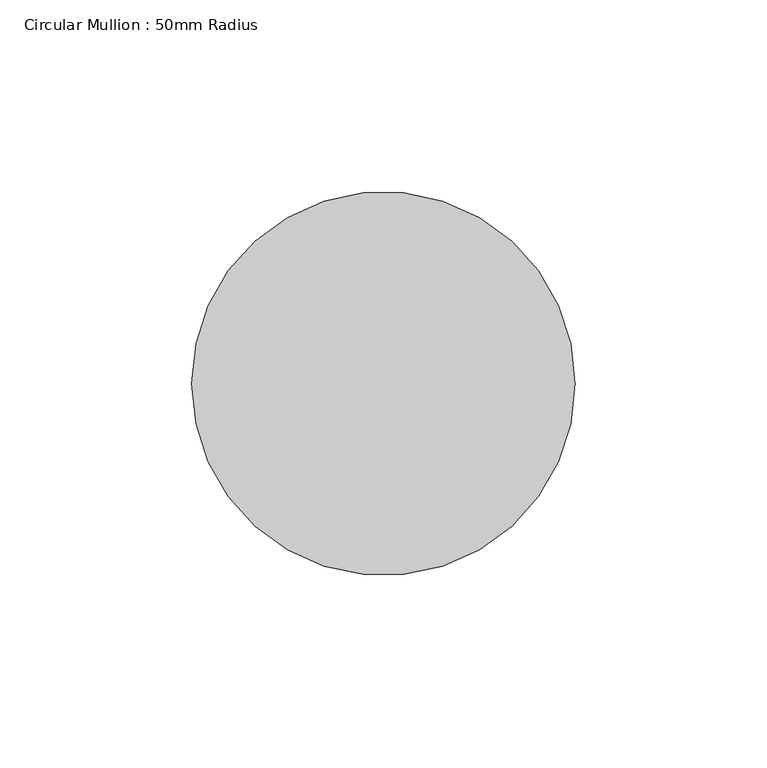
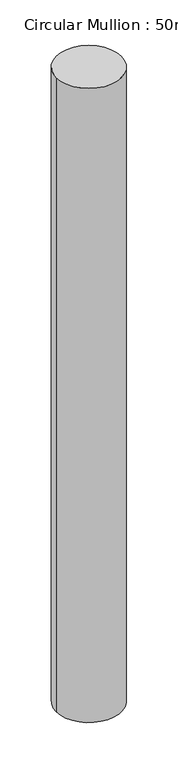
"""IFC4 building model written with IfcOpenShell, lengths in millimetres: member geometry, Circular Mullion : 50mm Radius."""

from ifc_helpers import new_model, si_unit, point, frame, origin, origin_2d, place, context, project, spatial, circle_curve, trimmed, segment, composite_curve, outline, extrude, source, transform, mapped, element, save


def circular_mullion_50mm_radius_1b65476c(model_context):
    return source(origin(), model_context, "Body", "SweptSolid", [
        extrude(outline(composite_curve([segment(trimmed(circle_curve(origin_2d(), 50.0), [point((50.0, 0.0))], [point((-50.0, 0.0))], False, "CARTESIAN"), True, "CONTINUOUS"), segment(trimmed(circle_curve(origin_2d(), 50.0), [point((-50.0, 0.0))], [point((50.0, 0.0))], False, "CARTESIAN"), True, "CONTINUOUS")], self_intersect=False)), frame((0.0, 0.0, -1031.8269354), z_axis=(0.0, 0.0, 1.0), x_axis=(1.0, 0.0, 0.0)), (0.0, 0.0, 1.0), 1031.8269354),
    ])


if __name__ == "__main__":
    model = new_model("IFC4")
    model_context = context("Model", 3, world=origin())
    ifc_project = project(units=[si_unit("LENGTHUNIT", "METRE", prefix="MILLI")], contexts=[model_context])
    site = spatial("IfcSite", under=ifc_project)
    building = spatial("IfcBuilding", under=site)
    placement = place(None, origin())
    circular_mullion_50mm_radius_shape = circular_mullion_50mm_radius_1b65476c(model_context)
    element("IfcMember", 1, ObjectType="Circular Mullion : 50mm Radius", at=placement, inside=building, context=model_context, shape_type="MappedRepresentation", body=[
        mapped(circular_mullion_50mm_radius_shape, transform((0.0, 0.0, 0.0), x_axis=(1.0, 0.0, 0.0), y_axis=(0.0, 1.0, 0.0), z_axis=(0.0, 0.0, 1.0))),
    ])
    save(model, "model.ifc")

# Revit data of these elements
# Type "Circular Mullion : 50mm Radius"
#   built-in parameter 1007350 = 0.164042 (stored number, unit not read)
# Element 1 (IfcMember, "Circular Mullion : 50mm Radius")
#   Materials on its faces: "Aluminium"
# Materials
#   "Aluminium": class "Metal", colour RGB 247 247 247, transparency 0, Description = "Aluminium 6061", Cost = 0
